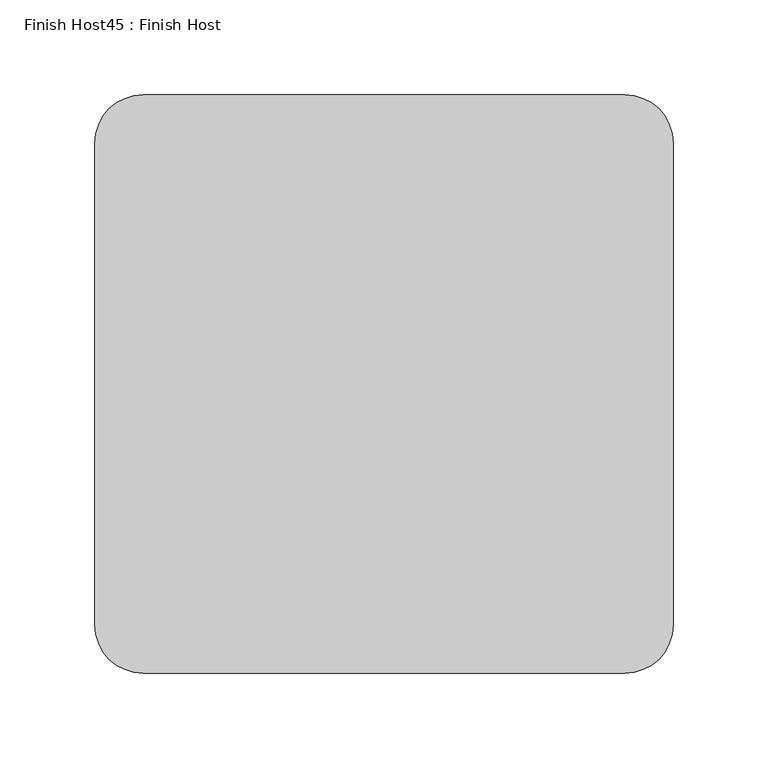
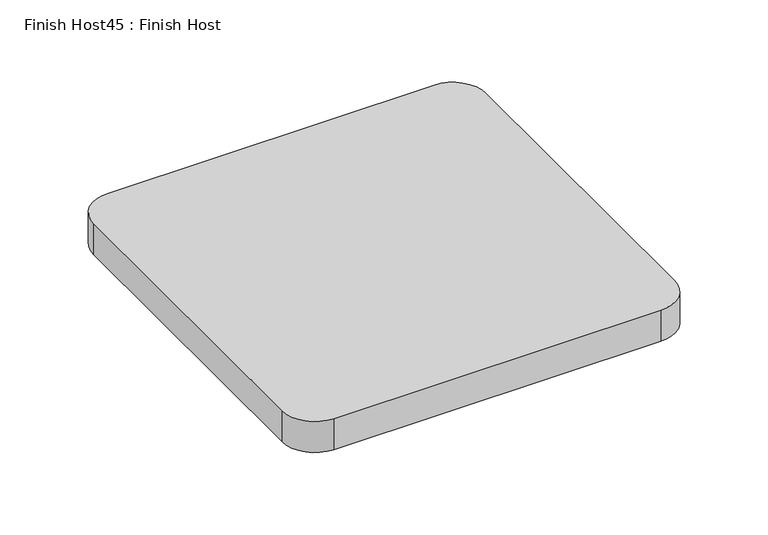
"""IFC4 building model written with IfcOpenShell, lengths in millimetres: proxy geometry, Finish Host45 : Finish Host."""

from ifc_helpers import new_model, si_unit, point, frame_2d, origin, origin_with_axes, place, context, project, spatial, polyline, circle_curve, trimmed, segment, composite_curve, outline, extrude, source, transform, mapped, element, save


def finish_host45_finish_host_9de219b9(model_context):
    return source(origin(), model_context, "Body", "SweptSolid", [
        extrude(outline(composite_curve([segment(polyline([(-15335.2939795, 14061.2419385), (-15335.2939795, 14315.2419385)]), True, "CONTINUOUS"), segment(trimmed(circle_curve(frame_2d((-15309.8939795, 14315.2419385)), 25.4), [point((-15335.2939795, 14315.2419385))], [point((-15309.8939795, 14340.6419385))], False, "CARTESIAN"), True, "CONTINUOUS"), segment(polyline([(-15309.8939795, 14340.6419385), (-15055.8939795, 14340.6419385)]), True, "CONTINUOUS"), segment(trimmed(circle_curve(frame_2d((-15055.8939795, 14315.2419385)), 25.4), [point((-15055.8939795, 14340.6419385))], [point((-15030.4939795, 14315.2419385))], False, "CARTESIAN"), True, "CONTINUOUS"), segment(polyline([(-15030.4939795, 14315.2419385), (-15030.4939795, 14061.2419385)]), True, "CONTINUOUS"), segment(trimmed(circle_curve(frame_2d((-15055.8939795, 14061.2419385)), 25.4), [point((-15030.4939795, 14061.2419385))], [point((-15055.8939795, 14035.8419385))], False, "CARTESIAN"), True, "CONTINUOUS"), segment(polyline([(-15055.8939795, 14035.8419385), (-15309.8939795, 14035.8419385)]), True, "CONTINUOUS"), segment(trimmed(circle_curve(frame_2d((-15309.8939795, 14061.2419385)), 25.4), [point((-15309.8939795, 14035.8419385))], [point((-15335.2939795, 14061.2419385))], False, "CARTESIAN"), True, "CONTINUOUS")], self_intersect=False)), origin_with_axes(), (0.0, 0.0, 1.0), 25.4),
    ])


if __name__ == "__main__":
    model = new_model("IFC4")
    model_context = context("Model", 3, world=origin())
    ifc_project = project(units=[si_unit("LENGTHUNIT", "METRE", prefix="MILLI")], contexts=[model_context])
    site = spatial("IfcSite", under=ifc_project)
    building = spatial("IfcBuilding", under=site)
    placement = place(None, origin())
    finish_host45_finish_host_shape = finish_host45_finish_host_9de219b9(model_context)
    element("IfcBuildingElementProxy", 1, Name="Finish Host45 : Finish Host", ObjectType="Finish Host45 : Finish Host", at=placement, inside=building, context=model_context, shape_type="MappedRepresentation", body=[
        mapped(finish_host45_finish_host_shape, transform((0.0, 0.0, 0.0), x_axis=(1.0, 0.0, 0.0), y_axis=(0.0, 1.0, 0.0), z_axis=(0.0, 0.0, 1.0))),
    ])
    save(model, "model.ifc")

# Revit data of these elements
# Type "Finish Host45 : Finish Host"
#   Countertop Material = none
# Element 1 (IfcBuildingElementProxy, "Finish Host45 : Finish Host")
#   Materials on its faces: "Thread - Teknion - Black"
# Materials
#   "Thread - Teknion - Black": class "Fabric", colour RGB 9 9 11, transparency 0, Model = "F206", Manufacturer = "Teknion Studio", URL = "http://www.teknion.com/", Description = "Fantasme Full Wool", Cost = 0
